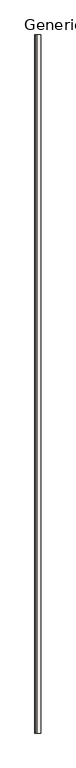
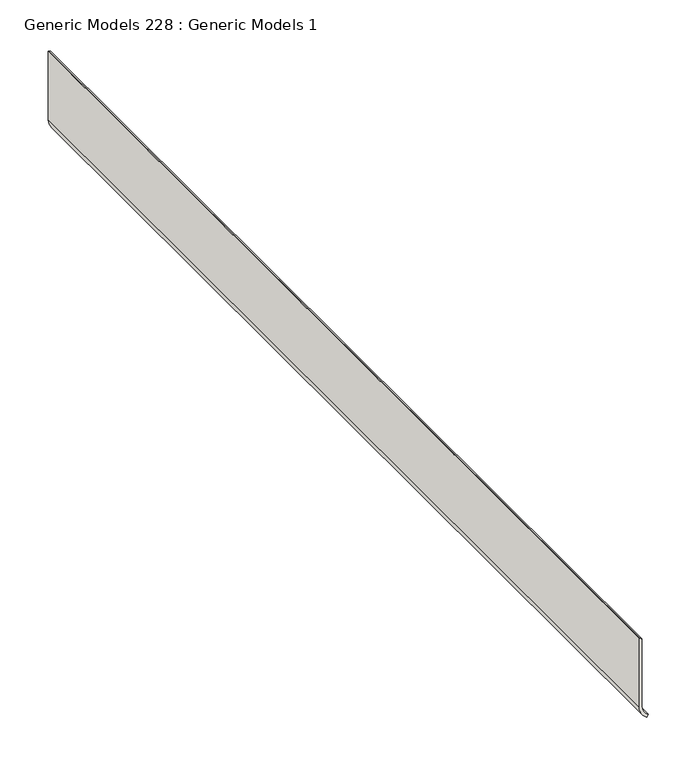
"""IFC4 building model written with IfcOpenShell, lengths in millimetres: wall geometry, Generic Models 228 : Generic Models 1."""

from ifc_helpers import new_model, si_unit, point, frame, frame_2d, origin, place, context, project, spatial, polyline, circle_curve, trimmed, segment, composite_curve, outline, extrude, source, transform, mapped, element, save


def generic_models_228_generic_models_1_2360532a(model_context):
    return source(origin(), model_context, "Body", "SweptSolid", [
        extrude(outline(composite_curve([segment(polyline([(101.6, 136363.075), (15.4496307, 136363.075)]), True, "CONTINUOUS"), segment(trimmed(circle_curve(frame_2d((15.4496307, 136380.9146968)), 17.8396968), [point((15.4496307, 136363.075))], [point((0.0, 136371.9948484))], False, "CARTESIAN"), True, "CONTINUOUS"), segment(polyline([(0.0, 136371.9948484), (2.7496307, 136373.5823484)]), True, "CONTINUOUS"), segment(trimmed(circle_curve(frame_2d((15.4496307, 136380.9146968)), 14.6646968), [point((2.7496307, 136373.5823484))], [point((15.4496307, 136366.25))], True, "CARTESIAN"), True, "CONTINUOUS"), segment(polyline([(15.4496307, 136366.25), (99.5131982, 136366.25)]), True, "CONTINUOUS"), segment(trimmed(circle_curve(frame_2d((99.5131982, 136364.1631982)), 2.0868018), [point((99.5131982, 136366.25))], [point((101.6, 136364.1631982))], False, "CARTESIAN"), True, "CONTINUOUS"), segment(polyline([(101.6, 136364.1631982), (101.6, 136363.075)]), True, "CONTINUOUS")], self_intersect=False)), frame((0.0, 0.0, 0.0), z_axis=(0.0, 1.0, 0.0), x_axis=(0.0, 0.0, 1.0)), (0.0, 0.0, 1.0), 1219.2),
    ])


if __name__ == "__main__":
    model = new_model("IFC4")
    model_context = context("Model", 3, world=origin())
    ifc_project = project(units=[si_unit("LENGTHUNIT", "METRE", prefix="MILLI")], contexts=[model_context])
    site = spatial("IfcSite", under=ifc_project)
    building = spatial("IfcBuilding", under=site)
    placement = place(None, origin())
    generic_models_228_generic_models_1_shape = generic_models_228_generic_models_1_2360532a(model_context)
    element("IfcWall", 1, ObjectType="Generic Models 228 : Generic Models 1", at=placement, inside=building, context=model_context, shape_type="MappedRepresentation", body=[
        mapped(generic_models_228_generic_models_1_shape, transform((0.0, 0.0, 0.0), x_axis=(1.0, 0.0, 0.0), y_axis=(0.0, 1.0, 0.0), z_axis=(0.0, 0.0, 1.0))),
    ])
    save(model, "model.ifc")

# Revit data of these elements
# Element 1 (IfcWall, "Generic Models 228 : Generic Models 1")
#   Materials on its faces: "WALL BASE AS SCHEDULED"
# Materials
#   "WALL BASE AS SCHEDULED": class "Generic", colour RGB 120 120 120, transparency 0, Cost = 0
